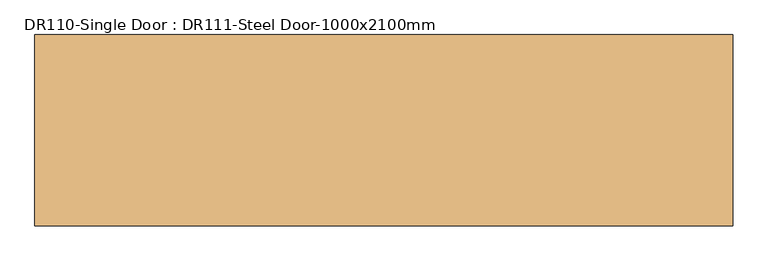
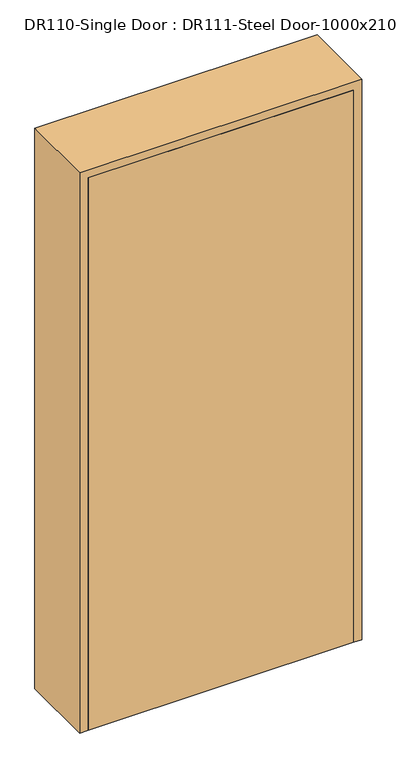
"""IFC4 building model written with IfcOpenShell, lengths in millimetres: door geometry, DR110-Single Door : DR111-Steel Door-1000x2100mm."""

from ifc_helpers import new_model, si_unit, origin, origin_with_axes, place, context, project, spatial, polyline, outline, extrude, faceted_brep, source, transform, mapped, element, save


def dr110_single_door_dr111_steel_door_1000x2100mm_c730d40a(model_context):
    return source(origin(), model_context, "Body", "SolidModel", [
        extrude(outline(polyline([(470.0, -137.0), (-470.0, -137.0), (-470.0, -102.0), (470.0, -102.0), (470.0, -137.0)])), origin_with_axes(), (0.0, 0.0, 1.0), 2070.0),
        faceted_brep([(470.0, -137.0, 0.0), (470.0, -102.0, 0.0), (450.0, -102.0, 0.0), (450.0, 102.0, 0.0), (470.0, 102.0, 0.0), (470.0, 137.0, 0.0), (500.0, 137.0, 0.0), (500.0, -137.0, 0.0), (500.0, -137.0, 2100.0), (-500.0, -137.0, 2100.0), (-500.0, -137.0, 0.0), (-470.0, -137.0, 0.0), (-470.0, -137.0, 2070.0), (470.0, -137.0, 2070.0), (500.0, 137.0, 2100.0), (470.0, 137.0, 2070.0), (-470.0, 137.0, 2070.0), (-470.0, 137.0, 0.0), (-500.0, 137.0, 0.0), (-500.0, 137.0, 2100.0), (470.0, 102.0, 2070.0), (450.0, 102.0, 2050.0), (-450.0, 102.0, 2050.0), (-450.0, 102.0, 0.0), (-470.0, 102.0, 0.0), (-470.0, 102.0, 2070.0), (450.0, -102.0, 2050.0), (470.0, -102.0, 2070.0), (-470.0, -102.0, 2070.0), (-470.0, -102.0, 0.0), (-450.0, -102.0, 0.0), (-450.0, -102.0, 2050.0)], [[[0, 1, 2, 3, 4, 5, 6, 7]], [[7, 8, 9, 10, 11, 12, 13, 0]], [[6, 14, 8, 7]], [[5, 15, 16, 17, 18, 19, 14, 6]], [[4, 20, 15, 5]], [[3, 21, 22, 23, 24, 25, 20, 4]], [[2, 26, 21, 3]], [[1, 27, 28, 29, 30, 31, 26, 2]], [[0, 13, 27, 1]], [[12, 11, 29, 28]], [[11, 10, 18, 17, 24, 23, 30, 29]], [[19, 18, 10, 9]], [[25, 24, 17, 16]], [[31, 30, 23, 22]], [[14, 19, 9, 8]], [[20, 25, 16, 15]], [[26, 31, 22, 21]], [[13, 12, 28, 27]]]),
    ])


if __name__ == "__main__":
    model = new_model("IFC4")
    model_context = context("Model", 3, world=origin())
    ifc_project = project(units=[si_unit("LENGTHUNIT", "METRE", prefix="MILLI")], contexts=[model_context])
    site = spatial("IfcSite", under=ifc_project)
    building = spatial("IfcBuilding", under=site)
    placement = place(None, origin())
    dr110_single_door_dr111_steel_door_1000x2100mm_shape = dr110_single_door_dr111_steel_door_1000x2100mm_c730d40a(model_context)
    element("IfcDoor", 1, ObjectType="DR110-Single Door : DR111-Steel Door-1000x2100mm", at=placement, inside=building, context=model_context, shape_type="MappedRepresentation", body=[
        mapped(dr110_single_door_dr111_steel_door_1000x2100mm_shape, transform((0.0, 0.0, 0.0), x_axis=(1.0, 0.0, 0.0), y_axis=(0.0, 1.0, 0.0), z_axis=(0.0, 0.0, 1.0))),
    ])
    save(model, "model.ifc")

# Revit data of these elements
# Type "DR110-Single Door : DR111-Steel Door-1000x2100mm"
#   Type Mark = "SD"
#   Analytic Construction = "<None>"
#   프레임 투영 외부. = 25 mm
#   프레임 투영 내부. = 25 mm
#   프레임 폭 = 75 mm
#   Height = 2100 mm
#   Width = 1000 mm
#   Define Thermal Properties by = 1
#   문 패널 = SD1 문 패널
#   문 프레임 = A04AQ098-00002_Steel Door_non FP_single
#   Function = (empty or 0)
#   Wall Closure = (empty or 0)
# Element 1 (IfcDoor, "DR110-Single Door : DR111-Steel Door-1000x2100mm")
#   Materials on its faces: "A04AQ098-00002_Steel Door_non FP_single", "SD1 문 패널"
# Materials
#   "SD1 문 패널": class "금속", colour RGB 247 247 247, transparency 0, Description = "STEEL DOOR (1000Wx2100H)"
#   "A04AQ098-00002_Steel Door_non FP_single": class "금속", colour RGB 247 247 247, transparency 0, Description = "Steel Door", W00) Work Master Code = "A04AQ098-00002", W01) Work Master_Lv1 = "Finishing Work", W02) Work Master_Lv2 = "Door & Window Work", W03) Work Master_Spec.1 = "Steel Door w/ Steel Frame", W04) Work Master_Spec.2 = "Fire Protective Rating: N/A, Single Door", W05) Work Master_Spec.3 = "w/ Hardware & Accessories", Cost = 0
